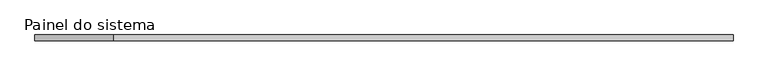
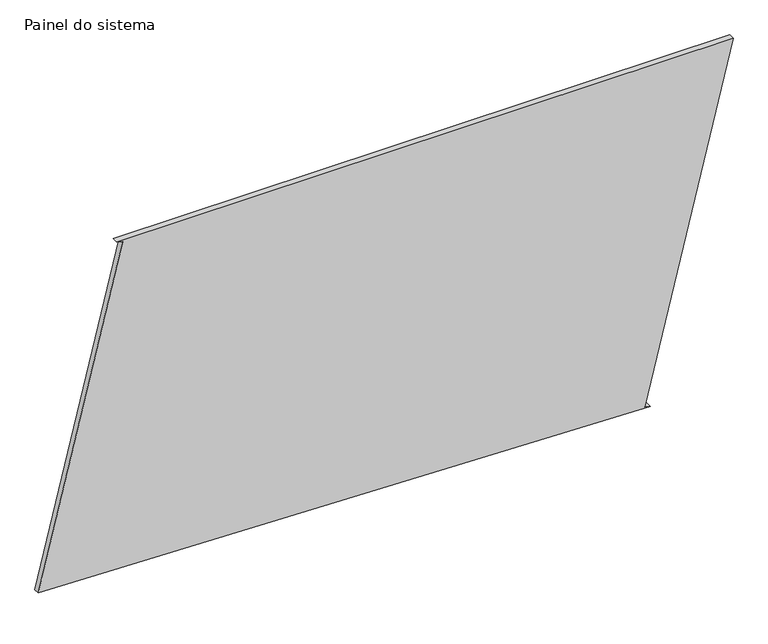
"""IFC4 building model written with IfcOpenShell, lengths in millimetres: plate geometry, Painel do sistema : Envidraçado."""

from ifc_helpers import new_model, si_unit, frame, origin, place, context, project, spatial, polyline, outline, extrude, source, transform, mapped, element, save


def painel_do_sistema_8bdf9dcd(model_context):
    return source(origin(), model_context, "Body", "SweptSolid", [
        extrude(outline(polyline([(0.0, 1126.9923638), (5.9765403, 1102.7172538), (1534.8005857, 1479.1142484), (1534.8005857, -1144.5905833), (1528.8240454, -1120.3154733), (71.4792665, -1479.1142484), (0.0, 1126.9923638)])), frame((0.0, 24.5, 0.0), z_axis=(0.0, 1.0, 0.0), x_axis=(0.0, 0.0, 1.0)), (0.0, 0.0, 1.0), 25.0),
    ])


if __name__ == "__main__":
    model = new_model("IFC4")
    model_context = context("Model", 3, world=origin())
    ifc_project = project(units=[si_unit("LENGTHUNIT", "METRE", prefix="MILLI")], contexts=[model_context])
    site = spatial("IfcSite", under=ifc_project)
    building = spatial("IfcBuilding", under=site)
    placement = place(None, origin())
    painel_do_sistema_shape = painel_do_sistema_8bdf9dcd(model_context)
    element("IfcPlate", 1, ObjectType="Painel do sistema : Envidraçado", at=placement, inside=building, context=model_context, shape_type="MappedRepresentation", body=[
        mapped(painel_do_sistema_shape, transform((0.0, 0.0, 0.0), x_axis=(1.0, 0.0, 0.0), y_axis=(0.0, 1.0, 0.0), z_axis=(0.0, 0.0, 1.0))),
    ])
    save(model, "model.ifc")

# Revit data of these elements
# Type "Painel do sistema : Envidraçado"
#   Construction Type Id = "GSP4R"
#   Analytic Construction = "Vidraça única Pilkington 1/8 pol"
#   Visual Light Transmittance = 0.9
#   Solar Heat Gain Coefficient = 0.86
#   Heat Transfer Coefficient (U) = 6.7069 W/(m²·K)
# Element 1 (IfcPlate, "Painel do sistema : Envidraçado")
#   Materials on its faces: "Vidro"
# Materials
#   "Vidro": class "Vidro", colour RGB 0 128 192, transparency 0.9, Description = "Vidro de sílica", Cost = 0
